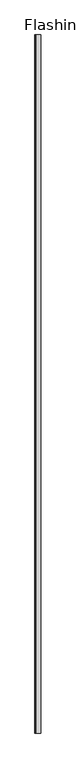
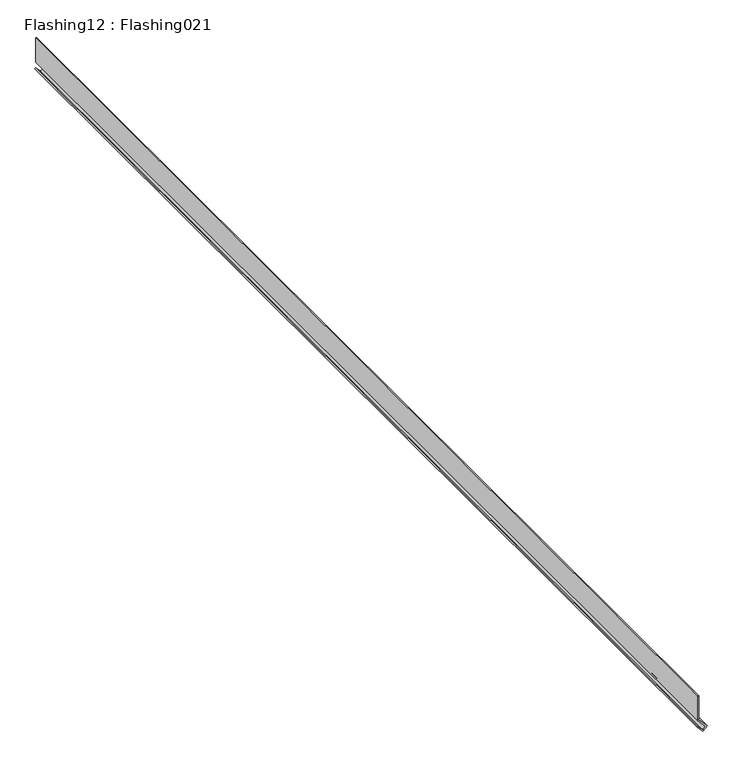
"""IFC4 building model written with IfcOpenShell, lengths in millimetres: proxy geometry, Flashing12 : Flashing021."""

from ifc_helpers import new_model, si_unit, frame, origin, place, context, project, spatial, polyline, outline, extrude, source, transform, mapped, element, save


def flashing12_flashing021_f64f48d8(model_context):
    return source(origin(), model_context, "Body", "SweptSolid", [
        extrude(outline(polyline([(43008.8710938, 16651.7480469), (42993.6445313, 16665.2148438), (42989.0546875, 16660.4316406), (42998.2304688, 16652.1347656), (42996.8890886, 16650.6512902), (42986.1852076, 16660.3298953), (42993.5310498, 16667.9852007), (43009.6286352, 16653.7480469), (43053.53125, 16653.7480469), (43053.53125, 16651.7480469), (43008.8710938, 16651.7480469)])), frame((0.0, 7982.1435673, 0.0), z_axis=(0.0, 1.0, 0.0), x_axis=(0.0, 0.0, 1.0)), (0.0, 0.0, 1.0), 2000.0),
    ])


if __name__ == "__main__":
    model = new_model("IFC4")
    model_context = context("Model", 3, world=origin())
    ifc_project = project(units=[si_unit("LENGTHUNIT", "METRE", prefix="MILLI")], contexts=[model_context])
    site = spatial("IfcSite", under=ifc_project)
    building = spatial("IfcBuilding", under=site)
    placement = place(None, origin())
    flashing12_flashing021_shape = flashing12_flashing021_f64f48d8(model_context)
    element("IfcBuildingElementProxy", 1, Name="Flashing12 : Flashing021", ObjectType="Flashing12 : Flashing021", at=placement, inside=building, context=model_context, shape_type="MappedRepresentation", body=[
        mapped(flashing12_flashing021_shape, transform((0.0, 0.0, 0.0), x_axis=(1.0, 0.0, 0.0), y_axis=(0.0, 1.0, 0.0), z_axis=(0.0, 0.0, 1.0))),
    ])
    save(model, "model.ifc")

# Revit data of these elements
# Type "Flashing12 : Flashing021"
#   NameOverride = "Flashing021"
# Element 1 (IfcBuildingElementProxy, "Flashing12 : Flashing021")
#   Materials on its faces: "16GA. COPPER BRAKE METAL FLASHING"
# Materials
#   "16GA. COPPER BRAKE METAL FLASHING": class "Unassigned", colour RGB 128 128 128, transparency 0, Cost = 0
